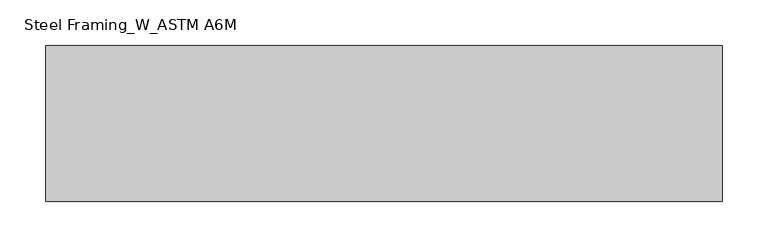
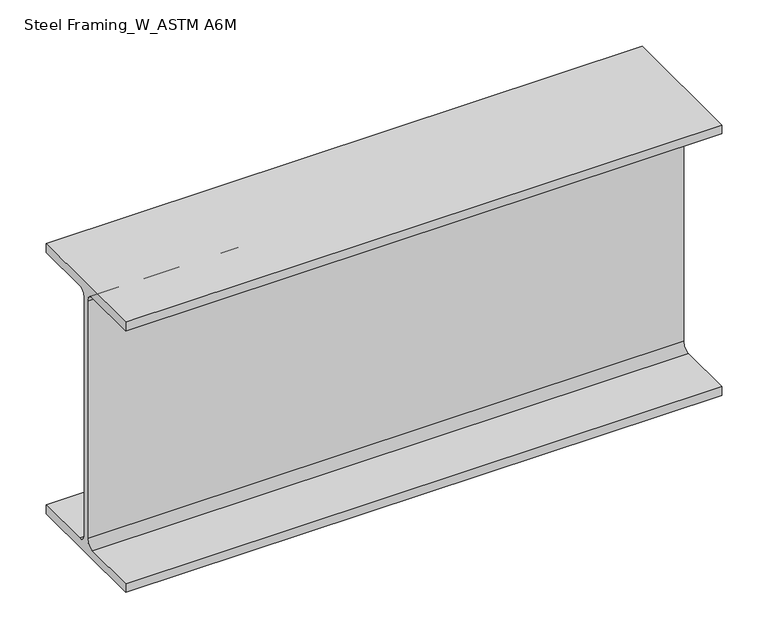
"""IFC4 building model written with IfcOpenShell, lengths in millimetres: beam geometry, Steel Framing_W_ASTM A6M : H_SB_AR_S02_W360x51_RG1."""

from ifc_helpers import new_model, si_unit, point, frame, frame_2d, origin, place, context, project, spatial, polyline, circle_curve, trimmed, segment, composite_curve, outline, extrude, source, transform, mapped, element, save


def steel_framing_w_astm_a6m_d5891017(model_context):
    return source(origin(), model_context, "Body", "SweptSolid", [
        extrude(outline(composite_curve([segment(polyline([(85.5, -166.4), (85.5, -178.0), (-85.5, -178.0), (-85.5, -166.4), (-13.72, -166.4)]), True, "CONTINUOUS"), segment(trimmed(circle_curve(frame_2d((-13.72, -156.3)), 10.1), [point((-13.72, -166.4))], [point((-3.62, -156.3))], True, "CARTESIAN"), True, "CONTINUOUS"), segment(polyline([(-3.62, -156.3), (-3.62, 156.3)]), True, "CONTINUOUS"), segment(trimmed(circle_curve(frame_2d((-13.72, 156.3)), 10.1), [point((-3.62, 156.3))], [point((-13.72, 166.4))], True, "CARTESIAN"), True, "CONTINUOUS"), segment(polyline([(-13.72, 166.4), (-85.5, 166.4), (-85.5, 178.0), (85.5, 178.0), (85.5, 166.4), (13.72, 166.4)]), True, "CONTINUOUS"), segment(trimmed(circle_curve(frame_2d((13.72, 156.3)), 10.1), [point((13.72, 166.4))], [point((3.62, 156.3))], True, "CARTESIAN"), True, "CONTINUOUS"), segment(polyline([(3.62, 156.3), (3.62, -156.3)]), True, "CONTINUOUS"), segment(trimmed(circle_curve(frame_2d((13.72, -156.3)), 10.1), [point((3.62, -156.3))], [point((13.72, -166.4))], True, "CARTESIAN"), True, "CONTINUOUS"), segment(polyline([(13.72, -166.4), (85.5, -166.4)]), True, "CONTINUOUS")], self_intersect=False)), frame((-493.6, 0.0, 0.0), z_axis=(1.0, 0.0, 0.0), x_axis=(0.0, 1.0, 0.0)), (0.0, 0.0, 1.0), 742.2),
    ])


if __name__ == "__main__":
    model = new_model("IFC4")
    model_context = context("Model", 3, world=origin())
    ifc_project = project(units=[si_unit("LENGTHUNIT", "METRE", prefix="MILLI")], contexts=[model_context])
    site = spatial("IfcSite", under=ifc_project)
    building = spatial("IfcBuilding", under=site)
    placement = place(None, origin())
    steel_framing_w_astm_a6m_shape = steel_framing_w_astm_a6m_d5891017(model_context)
    element("IfcBeam", 1, ObjectType="Steel Framing_W_ASTM A6M : H_SB_AR_S02_W360x51_RG1", at=placement, inside=building, context=model_context, shape_type="MappedRepresentation", body=[
        mapped(steel_framing_w_astm_a6m_shape, transform((0.0, 0.0, 0.0), x_axis=(1.0, 0.0, 0.0), y_axis=(0.0, 1.0, 0.0), z_axis=(0.0, 0.0, 1.0))),
    ])
    save(model, "model.ifc")

# Revit data of these elements
# Type "Steel Framing_W_ASTM A6M : H_SB_AR_S02_W360x51_RG1"
#   Type Mark = "RG1"
#   Section Name Key = "W14x34"
#   Width = 17.1 cm
#   Web Thickness = 0.724 cm
#   Web Fillet = 1.01 cm
#   Warping Constant = 287000.0 cm⁶
#   Torsional Moment of Inertia = 23.70 cm⁴
#   Section Area = 64.5 cm²
#   Plastic Modulus weak axis = 174.0 cm³
#   Plastic Modulus strong axis = 895.0 cm³
#   Perimeter = 1.36 m²/m
#   Nominal Weight = 51.00 kgf/m
#   Moment of Inertia weak axis = 970.00 cm⁴
#   Moment of Inertia strong axis = 14200.00 cm⁴
#   Height = 35.6 cm
#   Flange Thickness = 1.16 cm
#   Elastic Modulus weak axis = 113.0 cm³
#   Elastic Modulus strong axis = 796.0 cm³
#   Centroid Vertical = 17.8 cm
#   Centroid Horizontal = 8.55 cm
#   Length [instance default] = 1500 mm
#   Structural Material [instance default] = Steel, 45-345
#   Bolt Spacing = 0
#   Assembly Code = ""
# Element 1 (IfcBeam, "Steel Framing_W_ASTM A6M : H_SB_AR_S02_W360x51_RG1")
#   Materials on its faces: "Steel, 45-345"
# Materials
#   "Steel, 45-345": class "Metal", colour RGB 189 187 185, transparency 0, Description = "Steel 345 MPa", Cost = 0
